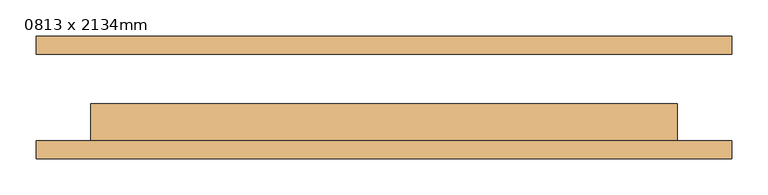
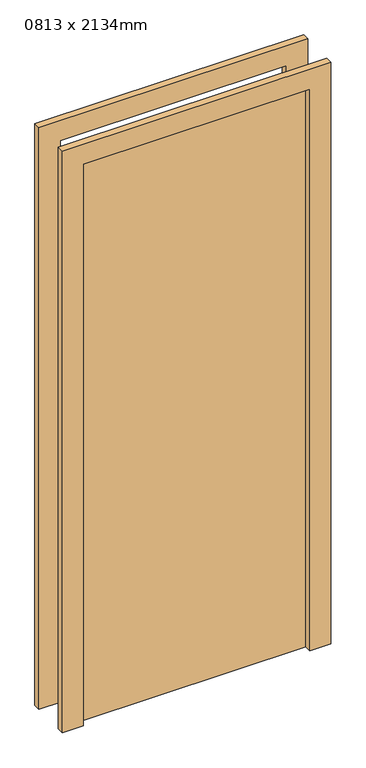
"""IFC4 building model written with IfcOpenShell, lengths in millimetres: door geometry, M_Folha única : 0813 x 2134mm."""

from ifc_helpers import new_model, si_unit, frame, origin, origin_with_axes, place, context, project, spatial, polyline, outline, extrude, source, transform, mapped, element, save


def door_0813_x_2134mm_8eb04c96(model_context):
    return source(origin(), model_context, "Body", "SweptSolid", [
        extrude(outline(polyline([(2210.0, -482.5), (0.0, -482.5), (0.0, -406.5), (2134.0, -406.5), (2134.0, 406.5), (0.0, 406.5), (0.0, 482.5), (2210.0, 482.5), (2210.0, -482.5)])), frame((0.0, -85.0, 0.0), z_axis=(0.0, 1.0, 0.0), x_axis=(0.0, 0.0, 1.0)), (0.0, 0.0, 1.0), 25.0),
        extrude(outline(polyline([(2210.0, 482.5), (2210.0, -482.5), (0.0, -482.5), (0.0, -406.5), (2134.0, -406.5), (2134.0, 406.5), (0.0, 406.5), (0.0, 482.5), (2210.0, 482.5)])), frame((0.0, 60.0, 0.0), z_axis=(0.0, 1.0, 0.0), x_axis=(0.0, 0.0, 1.0)), (0.0, 0.0, 1.0), 25.0),
        extrude(outline(polyline([(406.5, -9.0), (406.5, -60.0), (-406.5, -60.0), (-406.5, -9.0), (406.5, -9.0)])), origin_with_axes(), (0.0, 0.0, 1.0), 2134.0),
    ])


if __name__ == "__main__":
    model = new_model("IFC4")
    model_context = context("Model", 3, world=origin())
    ifc_project = project(units=[si_unit("LENGTHUNIT", "METRE", prefix="MILLI")], contexts=[model_context])
    site = spatial("IfcSite", under=ifc_project)
    building = spatial("IfcBuilding", under=site)
    placement = place(None, origin())
    door_0813_x_2134mm_shape = door_0813_x_2134mm_8eb04c96(model_context)
    element("IfcDoor", 1, ObjectType="M_Folha única : 0813 x 2134mm", at=placement, inside=building, context=model_context, shape_type="MappedRepresentation", body=[
        mapped(door_0813_x_2134mm_shape, transform((0.0, 0.0, 0.0), x_axis=(1.0, 0.0, 0.0), y_axis=(0.0, 1.0, 0.0), z_axis=(0.0, 0.0, 1.0))),
    ])
    save(model, "model.ifc")

# Revit data of these elements
# Type "M_Folha única : 0813 x 2134mm"
#   Type Mark = "24"
#   Construction Type Id = "MDOOR"
#   Analytic Construction = "Metal"
#   Thickness = 0.051 m
#   Thermal Resistance (R) = 0.270117 (m²·K)/W
#   Heat Transfer Coefficient (U) = 3.7021 W/(m²·K)
#   Height = 2.134 m
#   Projeção da apara externa = 0.025 m
#   Projeção da apara interna = 0.025 m
#   Largura da apara = 0.076 m
#   Width = 0.813 m
#   Define Thermal Properties by = 1
#   Define Thermal Properties by = 1
#   Material da porta = Porta - Painel
#   Material da moldura = Porta - Batente
#   Visual Light Transmittance = 0
#   Solar Heat Gain Coefficient = 0
#   Function = (empty or 0)
#   Wall Closure = (empty or 0)
# Element 1 (IfcDoor, "M_Folha única : 0813 x 2134mm")
#   Materials on its faces: "Porta - Batente", "Porta - Painel"
# Materials
#   "Porta - Painel": class "Madeira", colour RGB 210 159 95, transparency 0, Cost = 0
#   "Porta - Batente": class "Diversos", colour RGB 118 70 51, transparency 0, Cost = 0
